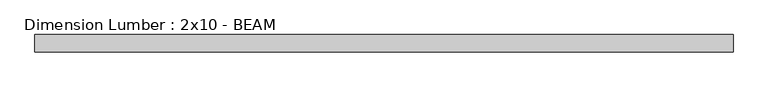
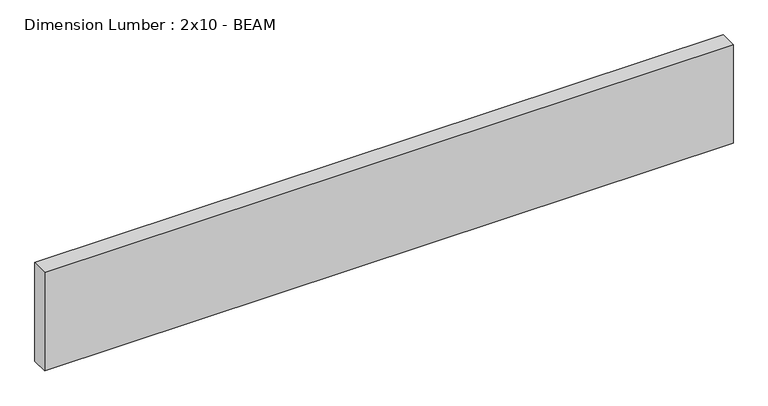
"""IFC4 building model written with IfcOpenShell, lengths in millimetres: beam geometry, Dimension Lumber : 2x10 - BEAM."""

from ifc_helpers import new_model, si_unit, frame, origin, place, context, project, spatial, polyline, outline, extrude, source, transform, mapped, element, save


def dimension_lumber_2x10_beam_b9c4c0be(model_context):
    return source(origin(), model_context, "Body", "SweptSolid", [
        extrude(outline(polyline([(774.7, 19.05), (774.7, -19.05), (-774.6999994, -19.05), (-774.6999994, 19.05), (774.7, 19.05)])), frame((0.0, 0.0, -117.475), z_axis=(0.0, 0.0, 1.0), x_axis=(1.0, 0.0, 0.0)), (0.0, 0.0, 1.0), 234.95),
    ])


if __name__ == "__main__":
    model = new_model("IFC4")
    model_context = context("Model", 3, world=origin())
    ifc_project = project(units=[si_unit("LENGTHUNIT", "METRE", prefix="MILLI")], contexts=[model_context])
    site = spatial("IfcSite", under=ifc_project)
    building = spatial("IfcBuilding", under=site)
    placement = place(None, origin())
    dimension_lumber_2x10_beam_shape = dimension_lumber_2x10_beam_b9c4c0be(model_context)
    element("IfcBeam", 1, ObjectType="Dimension Lumber : 2x10 - BEAM", at=placement, inside=building, context=model_context, shape_type="MappedRepresentation", body=[
        mapped(dimension_lumber_2x10_beam_shape, transform((0.0, 0.0, 0.0), x_axis=(1.0, 0.0, 0.0), y_axis=(0.0, 1.0, 0.0), z_axis=(0.0, 0.0, 1.0))),
    ])
    save(model, "model.ifc")

# Revit data of these elements
# Type "Dimension Lumber : 2x10 - BEAM"
#   Assembly Code = "B10"
#   A = 0.0755556 SF
#   Length [instance default] = 5' - 0"
#   b = 0' - 1 1/2"
#   d = 0' - 9 1/4"
#   Structural Material = (3) SISTERED 2X10s AT BEAM
# Element 1 (IfcBeam, "Dimension Lumber : 2x10 - BEAM")
#   Materials on its faces: "(3) SISTERED 2X10s AT BEAM"
# Materials
#   "(3) SISTERED 2X10s AT BEAM": class "Wood", colour RGB 234 198 147, transparency 0, Description = "Pinus Echinata", Cost = 0
